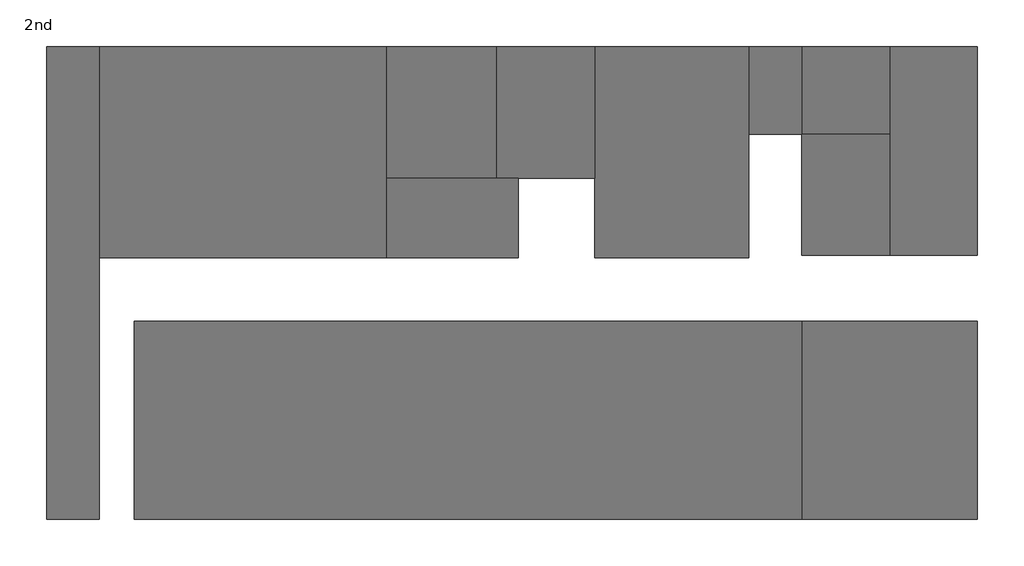
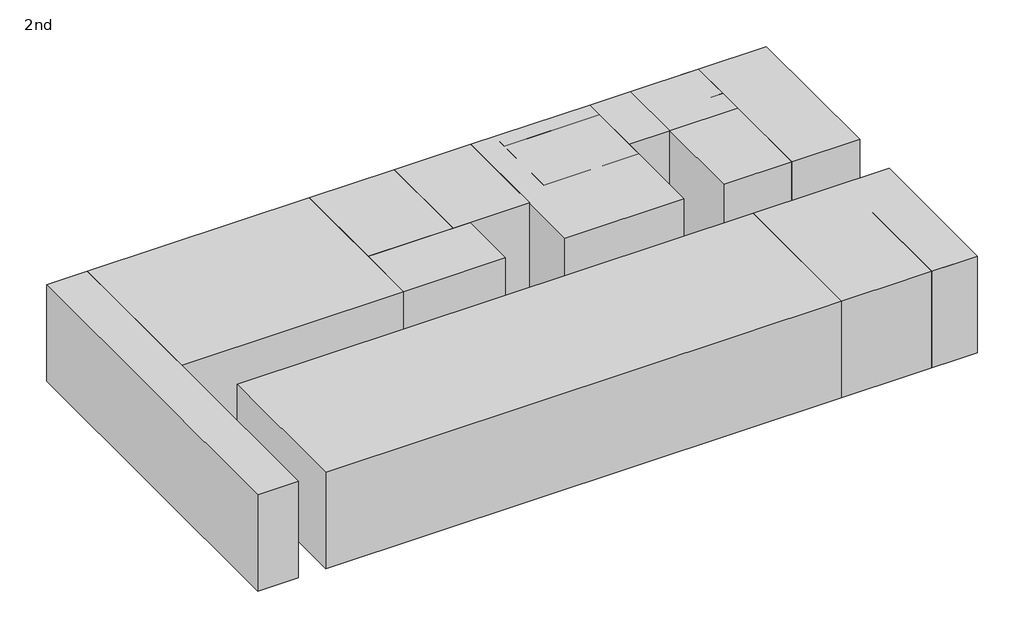
# One storey: 17 proxies.
"""IFC4 building model written with IfcOpenShell, lengths in millimetres."""

import ifcopenshell
import ifcopenshell.guid

model = None  # the IFC model being written
_history = None  # IfcOwnerHistory: only IFC2X3 demands one
_inside = {}  # id of a spatial element -> (the spatial element, [elements in it])
_under = {}  # id of a project, library or spatial element -> (it, [spatial elements below it])
_declared = {}  # id of a project -> (the project, [libraries it declares])
_typed = {}  # id of a type object -> (the type object, [elements of that type])
_made_of = {}  # id of a material, layer set ... -> (it, [elements and type objects made of it])


def new_model(schema):
    """Start an empty IFC model of exactly this schema.

    Asked for "IFC4X3", IfcOpenShell would pick the latest addendum, in which some entities
    have other attributes; the version numbers below select the first issue.
    IFC2X3 requires an IfcOwnerHistory on every rooted entity: one is made here for all.
    """
    global model, _history
    if schema == "IFC4X3":
        model = ifcopenshell.file(schema_version=(4, 3, 0, 0))
    else:
        model = ifcopenshell.file(schema=schema)
    _inside.clear()
    _under.clear()
    _declared.clear()
    _typed.clear()
    _made_of.clear()
    _history = None
    if model.schema == "IFC2X3":
        org = make("IfcOrganization", Name="unknown")
        user = make(
            "IfcPersonAndOrganization",
            ThePerson=make("IfcPerson", FamilyName="unknown"),
            TheOrganization=org,
        )
        app = make(
            "IfcApplication",
            ApplicationDeveloper=org,
            Version="unknown",
            ApplicationFullName="unknown",
            ApplicationIdentifier="unknown",
        )
        _history = make(
            "IfcOwnerHistory",
            OwningUser=user,
            OwningApplication=app,
            ChangeAction="ADDED",
            CreationDate=0,
        )
    return model


def make(cls, **values):
    """One entity of the class cls with the attributes given. An attribute that is None is left unset."""
    return model.create_entity(
        cls, **{name: value for name, value in values.items() if value is not None}
    )


def rooted(cls, **values):
    """An entity with a GlobalId (a new one), such as an element, a storey or a relation."""
    return make(cls, GlobalId=ifcopenshell.guid.new(), OwnerHistory=_history, **values)


def si_unit(unit_type, name, prefix=None):
    """IfcSIUnit, for example si_unit("LENGTHUNIT", "METRE", prefix="MILLI")."""
    return make("IfcSIUnit", UnitType=unit_type, Prefix=prefix, Name=name)


def assignment(units):
    """IfcUnitAssignment: the units of a project."""
    return None if units is None else make("IfcUnitAssignment", Units=units)


def point(xyz):
    """IfcCartesianPoint."""
    return None if xyz is None else make("IfcCartesianPoint", Coordinates=xyz)


def direction(xyz):
    """IfcDirection."""
    return None if xyz is None else make("IfcDirection", DirectionRatios=xyz)


def frame(location, z_axis=None, x_axis=None):
    """IfcAxis2Placement3D, a coordinate frame: its origin and axes. An axis left out is left unset."""
    return make(
        "IfcAxis2Placement3D",
        Location=point(location),
        Axis=direction(z_axis),
        RefDirection=direction(x_axis),
    )


def origin():
    """The frame at (0, 0, 0) with its axes left unset."""
    return frame((0.0, 0.0, 0.0))


def origin_with_axes():
    """The frame at (0, 0, 0) with the z axis (0, 0, 1) and the x axis (1, 0, 0) written out."""
    return frame((0.0, 0.0, 0.0), z_axis=(0.0, 0.0, 1.0), x_axis=(1.0, 0.0, 0.0))


def place(relative_to, where):
    """IfcLocalPlacement: puts the frame where relative to a parent placement (None: the world)."""
    return make(
        "IfcLocalPlacement", PlacementRelTo=relative_to, RelativePlacement=where
    )


def context(
    kind, dimensions, precision=None, world=None, true_north=None, identifier=None
):
    """IfcGeometricRepresentationContext, for example the 3D "Model" context."""
    return make(
        "IfcGeometricRepresentationContext",
        ContextIdentifier=identifier,
        ContextType=kind,
        CoordinateSpaceDimension=dimensions,
        Precision=precision,
        WorldCoordinateSystem=world,
        TrueNorth=true_north,
    )


def project(units=None, contexts=None):
    """IfcProject with its units and contexts."""
    return rooted(
        "IfcProject",
        Name="project",
        RepresentationContexts=contexts,
        UnitsInContext=assignment(units),
    )


def spatial(cls, under=None, at=None, **own):
    """A site, building, storey or space (cls), placed at a placement, below another one or the project."""
    s = rooted(cls, ObjectPlacement=at, **own)
    if under is not None:
        _under.setdefault(under.id(), (under, []))[1].append(s)
    return s


def polyline(points):
    """IfcPolyline through the points."""
    return make("IfcPolyline", Points=[point(p) for p in points])


def outline(outer, holes=None, kind="AREA"):
    """IfcArbitraryClosedProfileDef: a profile drawn as a closed curve; with holes, ...WithVoids."""
    if holes is None:
        return make("IfcArbitraryClosedProfileDef", ProfileType=kind, OuterCurve=outer)
    return make(
        "IfcArbitraryProfileDefWithVoids",
        ProfileType=kind,
        OuterCurve=outer,
        InnerCurves=holes,
    )


def extrude(swept, where, along, depth):
    """IfcExtrudedAreaSolid: the profile swept, set in the frame where, extruded along a direction by depth."""
    return make(
        "IfcExtrudedAreaSolid",
        SweptArea=swept,
        Position=where,
        ExtrudedDirection=direction(along),
        Depth=depth,
    )


def shape(context_of_items, identifier, shape_type, items):
    """IfcShapeRepresentation: the items that make up one representation, for example the "Body"."""
    return make(
        "IfcShapeRepresentation",
        ContextOfItems=context_of_items,
        RepresentationIdentifier=identifier,
        RepresentationType=shape_type,
        Items=items,
    )


def source(mapping_origin, context_of_items, identifier, shape_type, items):
    """IfcRepresentationMap: a shape defined once, which mapped items show again and again."""
    return make(
        "IfcRepresentationMap",
        MappingOrigin=mapping_origin,
        MappedRepresentation=shape(context_of_items, identifier, shape_type, items),
    )


def transform(
    local_origin,
    x_axis=None,
    y_axis=None,
    z_axis=None,
    scale=None,
    scale2=None,
    scale3=None,
    uniform=True,
):
    """IfcCartesianTransformationOperator3D, or its non-uniform kind. x_axis, y_axis, z_axis: its Axis1, 2, 3."""
    if uniform:
        return make(
            "IfcCartesianTransformationOperator3D",
            Axis1=direction(x_axis),
            Axis2=direction(y_axis),
            LocalOrigin=point(local_origin),
            Scale=scale,
            Axis3=direction(z_axis),
        )
    return make(
        "IfcCartesianTransformationOperator3DnonUniform",
        Axis1=direction(x_axis),
        Axis2=direction(y_axis),
        LocalOrigin=point(local_origin),
        Scale=scale,
        Axis3=direction(z_axis),
        Scale2=scale2,
        Scale3=scale3,
    )


def mapped(mapping_source, mapping_target):
    """IfcMappedItem: shows the shape of a source again, moved by a transform."""
    return make(
        "IfcMappedItem", MappingSource=mapping_source, MappingTarget=mapping_target
    )


def made_of(thing, what):
    """Note that an element or type object is made of a material, layer set ...; save() writes the relation."""
    if what is not None:
        _made_of.setdefault(what.id(), (what, []))[1].append(thing)
    return thing


def element(
    cls,
    number,
    at=None,
    inside=None,
    cuts=None,
    type_object=None,
    material=None,
    context=None,
    identifier="Body",
    shape_type=None,
    held_by="IfcProductDefinitionShape",
    body=None,
    shapes=None,
    **own,
):
    """One element of the class cls, such as IfcWall. Its Tag is "e" and its number.

    at: its placement. inside: the storey or other place that contains it. cuts: it is an
    opening in that element (IfcRelVoidsElement). A single representation is given by context,
    identifier, shape_type and body (its items); several are given by shapes. held_by: the class
    of the entity that holds the representations. save() writes the other relations.
    """
    e = rooted(cls, Tag="e%d" % number, ObjectPlacement=at, **own)
    if body is not None:
        shapes = [shape(context, identifier, shape_type, body)]
    if shapes is not None:
        e.Representation = make(held_by, Representations=shapes)
    if inside is not None:
        _inside.setdefault(inside.id(), (inside, []))[1].append(e)
    if cuts is not None:
        rooted(
            "IfcRelVoidsElement", RelatingBuildingElement=cuts, RelatedOpeningElement=e
        )
    if type_object is not None:
        _typed.setdefault(type_object.id(), (type_object, []))[1].append(e)
    return made_of(e, material)


def aggregate(whole, parts):
    """IfcRelAggregates: a whole, such as a stair, and the parts it consists of."""
    return rooted("IfcRelAggregates", RelatingObject=whole, RelatedObjects=parts)


def save(model, path):
    """Write the relations noted so far, then the file.

    IfcRelAggregates (storeys below a building ...), IfcRelContainedInSpatialStructure (elements
    in a storey), IfcRelDefinesByType, IfcRelAssociatesMaterial and IfcRelDeclares: one each for
    every whole, place, type object, material and project.
    """
    for whole, parts in _under.values():
        aggregate(whole, parts)
    for where, things in _inside.values():
        rooted(
            "IfcRelContainedInSpatialStructure",
            RelatedElements=things,
            RelatingStructure=where,
        )
    for kind, things in _typed.values():
        rooted("IfcRelDefinesByType", RelatedObjects=things, RelatingType=kind)
    for what, things in _made_of.values():
        rooted("IfcRelAssociatesMaterial", RelatedObjects=things, RelatingMaterial=what)
    for by, libraries in _declared.values():
        rooted("IfcRelDeclares", RelatingContext=by, RelatedDefinitions=libraries)
    model.write(path)


def space_planning_box_space_planning_box_5634f436(model_context):
    return source(origin(), model_context, "Body", "SweptSolid", [
        extrude(outline(polyline([(1350.0, 3000.0), (1350.0, -3000.0), (-1350.0, -3000.0), (-1350.0, 3000.0), (1350.0, 3000.0)])), origin_with_axes(), (0.0, 0.0, 1.0), 6000.0),
    ])


def space_planning_box_space_planning_box_71e2440f(model_context):
    return source(origin(), model_context, "Body", "SweptSolid", [
        extrude(outline(polyline([(500.0, 1250.0), (500.0, -1250.0), (-500.0, -1250.0), (-500.0, 1250.0), (500.0, 1250.0)])), origin_with_axes(), (0.0, 0.0, 1.0), 6000.0),
    ])


def space_planning_box_space_planning_box_ce7d2093(model_context):
    return source(origin(), model_context, "Body", "SweptSolid", [
        extrude(outline(polyline([(4500.0, 15175.0), (4500.0, -15175.0), (-4500.0, -15175.0), (-4500.0, 15175.0), (4500.0, 15175.0)])), origin_with_axes(), (0.0, 0.0, 1.0), 6000.0),
    ])


def space_planning_box_space_planning_box_c2e9f8fb(model_context):
    return source(origin(), model_context, "Body", "SweptSolid", [
        extrude(outline(polyline([(4800.0, 6525.0), (4800.0, -6525.0), (-4800.0, -6525.0), (-4800.0, 6525.0), (4800.0, 6525.0)])), origin_with_axes(), (0.0, 0.0, 1.0), 6000.0),
    ])


def space_planning_box_space_planning_box_44ef6168(model_context):
    return source(origin(), model_context, "Body", "SweptSolid", [
        extrude(outline(polyline([(2500.0, 3000.0), (2500.0, -3000.0), (-2500.0, -3000.0), (-2500.0, 3000.0), (2500.0, 3000.0)])), origin_with_axes(), (0.0, 0.0, 1.0), 6000.0),
    ])


def space_planning_box_space_planning_box_4d084078(model_context):
    return source(origin(), model_context, "Body", "SweptSolid", [
        extrude(outline(polyline([(4000.0, 4500.0), (4000.0, -4500.0), (-4000.0, -4500.0), (-4000.0, 4500.0), (4000.0, 4500.0)])), origin_with_axes(), (0.0, 0.0, 1.0), 6000.0),
    ])


def space_planning_box_space_planning_box_072414e0(model_context):
    return source(origin(), model_context, "Body", "SweptSolid", [
        extrude(outline(polyline([(3500.0, 4800.0), (3500.0, -4800.0), (-3500.0, -4800.0), (-3500.0, 4800.0), (3500.0, 4800.0)])), origin_with_axes(), (0.0, 0.0, 1.0), 6000.0),
    ])


def space_planning_box_space_planning_box_34e84c64(model_context):
    return source(origin(), model_context, "Body", "SweptSolid", [
        extrude(outline(polyline([(2750.0, 2000.0), (2750.0, -2000.0), (-2750.0, -2000.0), (-2750.0, 2000.0), (2750.0, 2000.0)])), origin_with_axes(), (0.0, 0.0, 1.0), 6000.0),
    ])


def space_planning_box_space_planning_box_7bff30ad(model_context):
    return source(origin(), model_context, "Body", "SweptSolid", [
        extrude(outline(polyline([(2000.0, 2000.0), (2000.0, -2000.0), (-2000.0, -2000.0), (-2000.0, 2000.0), (2000.0, 2000.0)])), origin_with_axes(), (0.0, 0.0, 1.0), 6000.0),
    ])


def space_planning_box_space_planning_box_03407eb8(model_context):
    return source(origin(), model_context, "Body", "SweptSolid", [
        extrude(outline(polyline([(1200.0, 10750.0), (1200.0, -10750.0), (-1200.0, -10750.0), (-1200.0, 10750.0), (1200.0, 10750.0)])), origin_with_axes(), (0.0, 0.0, 1.0), 6000.0),
    ])


def space_planning_box_space_planning_box_3a820573(model_context):
    return source(origin(), model_context, "Body", "SweptSolid", [
        extrude(outline(polyline([(2000.0, 4750.0), (2000.0, -4750.0), (-2000.0, -4750.0), (-2000.0, 4750.0), (2000.0, 4750.0)])), origin_with_axes(), (0.0, 0.0, 1.0), 6000.0),
    ])


def space_planning_box_space_planning_box_8af91fed(model_context):
    return source(origin(), model_context, "Body", "SweptSolid", [
        extrude(outline(polyline([(2250.0, 3000.0), (2250.0, -3000.0), (-2250.0, -3000.0), (-2250.0, 3000.0), (2250.0, 3000.0)])), origin_with_axes(), (0.0, 0.0, 1.0), 6000.0),
    ])


def space_planning_box_space_planning_box_837d2e24(model_context):
    return source(origin(), model_context, "Body", "SweptSolid", [
        extrude(outline(polyline([(1800.0, 3000.0), (1800.0, -3000.0), (-1800.0, -3000.0), (-1800.0, 3000.0), (1800.0, 3000.0)])), origin_with_axes(), (0.0, 0.0, 1.0), 6000.0),
    ])


def space_planning_box_space_planning_box_47b98be1(model_context):
    return source(origin(), model_context, "Body", "SweptSolid", [
        extrude(outline(polyline([(1200.0, 2000.0), (1200.0, -2000.0), (-1200.0, -2000.0), (-1200.0, 2000.0), (1200.0, 2000.0)])), origin_with_axes(), (0.0, 0.0, 1.0), 6000.0),
    ])


def space_planning_box_space_planning_box_a556ef48(model_context):
    return source(origin(), model_context, "Body", "SweptSolid", [
        extrude(outline(polyline([(500.0, 2800.0), (500.0, -2800.0), (-500.0, -2800.0), (-500.0, 2800.0), (500.0, 2800.0)])), origin_with_axes(), (0.0, 0.0, 1.0), 6000.0),
    ])


def space_planning_box_space_planning_box_c1734578(model_context):
    return source(origin(), model_context, "Body", "SweptSolid", [
        extrude(outline(polyline([(2800.0, 2500.0), (2800.0, -2500.0), (-2800.0, -2500.0), (-2800.0, 2500.0), (2800.0, 2500.0)])), origin_with_axes(), (0.0, 0.0, 1.0), 6000.0),
    ])


model = new_model("IFC4")

# Units and contexts
model_context = context("Model", 3, world=origin())
ifc_project = project(units=[si_unit("LENGTHUNIT", "METRE", prefix="MILLI")], contexts=[model_context])

# Site, building, storey
site = spatial("IfcSite", under=ifc_project)
building = spatial("IfcBuilding", under=site)
storey = spatial("IfcBuildingStorey", under=building, Name="2nd", Elevation=14000.0)

# Proxies
placement = place(None, origin())
space_planning_box_space_planning_box_shape = space_planning_box_space_planning_box_5634f436(model_context)
element("IfcBuildingElementProxy", 1, Name="Space Planning Box : Space Planning Box", ObjectType="Space Planning Box : Space Planning Box", at=placement, inside=storey, context=model_context, shape_type="MappedRepresentation", body=[
    mapped(space_planning_box_space_planning_box_shape, transform((48750.0, 154250.0, 14000.0), x_axis=(1.0, 0.0, 0.0), y_axis=(0.0, 1.0, 0.0), z_axis=(0.0, 0.0, 1.0))),
])
space_planning_box_space_planning_box_2_shape = space_planning_box_space_planning_box_71e2440f(model_context)
element("IfcBuildingElementProxy", 2, Name="Space Planning Box : Space Planning Box", ObjectType="Space Planning Box : Space Planning Box", at=placement, inside=storey, context=model_context, shape_type="MappedRepresentation", body=[
    mapped(space_planning_box_space_planning_box_2_shape, transform((45600.0, 171500.0, 14000.0), x_axis=(1.0, 0.0, 0.0), y_axis=(0.0, 1.0, 0.0), z_axis=(0.0, 0.0, 1.0))),
])
space_planning_box_space_planning_box_3_shape = space_planning_box_space_planning_box_ce7d2093(model_context)
element("IfcBuildingElementProxy", 3, Name="Space Planning Box : Space Planning Box", ObjectType="Space Planning Box : Space Planning Box", at=placement, inside=storey, context=model_context, shape_type="MappedRepresentation", body=[
    mapped(space_planning_box_space_planning_box_3_shape, transform((26925.0, 155750.0, 14000.0), x_axis=(0.0, -1.0, 0.0), y_axis=(1.0, 0.0, 0.0), z_axis=(0.0, 0.0, 1.0))),
])
space_planning_box_space_planning_box_4_shape = space_planning_box_space_planning_box_c2e9f8fb(model_context)
element("IfcBuildingElementProxy", 4, Name="Space Planning Box : Space Planning Box", ObjectType="Space Planning Box : Space Planning Box", at=placement, inside=storey, context=model_context, shape_type="MappedRepresentation", body=[
    mapped(space_planning_box_space_planning_box_4_shape, transform((16675.0, 167950.0, 14000.0), x_axis=(0.0, -1.0, 0.0), y_axis=(1.0, 0.0, 0.0), z_axis=(0.0, 0.0, 1.0))),
])
space_planning_box_space_planning_box_5_shape = space_planning_box_space_planning_box_44ef6168(model_context)
element("IfcBuildingElementProxy", 5, Name="Space Planning Box : Space Planning Box", ObjectType="Space Planning Box : Space Planning Box", at=placement, inside=storey, context=model_context, shape_type="MappedRepresentation", body=[
    mapped(space_planning_box_space_planning_box_5_shape, transform((25700.0, 169750.0, 14000.0), x_axis=(1.0, 0.0, 0.0), y_axis=(0.0, 1.0, 0.0), z_axis=(0.0, 0.0, 1.0))),
])
space_planning_box_space_planning_box_6_shape = space_planning_box_space_planning_box_4d084078(model_context)
element("IfcBuildingElementProxy", 6, Name="Space Planning Box : Space Planning Box", ObjectType="Space Planning Box : Space Planning Box", at=placement, inside=storey, context=model_context, shape_type="MappedRepresentation", body=[
    mapped(space_planning_box_space_planning_box_6_shape, transform((46100.0, 155750.0, 14000.0), x_axis=(1.0, 0.0, 0.0), y_axis=(0.0, 1.0, 0.0), z_axis=(0.0, 0.0, 1.0))),
])
space_planning_box_space_planning_box_7_shape = space_planning_box_space_planning_box_072414e0(model_context)
element("IfcBuildingElementProxy", 7, Name="Space Planning Box : Space Planning Box", ObjectType="Space Planning Box : Space Planning Box", at=placement, inside=storey, context=model_context, shape_type="MappedRepresentation", body=[
    mapped(space_planning_box_space_planning_box_7_shape, transform((36200.0, 167950.0, 14000.0), x_axis=(1.0, 0.0, 0.0), y_axis=(0.0, 1.0, 0.0), z_axis=(0.0, 0.0, 1.0))),
])
space_planning_box_space_planning_box_8_shape = space_planning_box_space_planning_box_34e84c64(model_context)
element("IfcBuildingElementProxy", 8, Name="Space Planning Box : Space Planning Box", ObjectType="Space Planning Box : Space Planning Box", at=placement, inside=storey, context=model_context, shape_type="MappedRepresentation", body=[
    mapped(space_planning_box_space_planning_box_8_shape, transform((44100.0, 166000.0, 14000.0), x_axis=(0.0, -1.0, 0.0), y_axis=(1.0, 0.0, 0.0), z_axis=(0.0, 0.0, 1.0))),
])
space_planning_box_space_planning_box_9_shape = space_planning_box_space_planning_box_7bff30ad(model_context)
element("IfcBuildingElementProxy", 9, Name="Space Planning Box : Space Planning Box", ObjectType="Space Planning Box : Space Planning Box", at=placement, inside=storey, context=model_context, shape_type="MappedRepresentation", body=[
    mapped(space_planning_box_space_planning_box_9_shape, transform((44100.0, 170750.0, 14000.0), x_axis=(1.0, 0.0, 0.0), y_axis=(0.0, 1.0, 0.0), z_axis=(0.0, 0.0, 1.0))),
])
space_planning_box_space_planning_box_10_shape = space_planning_box_space_planning_box_03407eb8(model_context)
element("IfcBuildingElementProxy", 10, Name="Space Planning Box : Space Planning Box", ObjectType="Space Planning Box : Space Planning Box", at=placement, inside=storey, context=model_context, shape_type="MappedRepresentation", body=[
    mapped(space_planning_box_space_planning_box_10_shape, transform((8950.0, 162000.0, 14000.0), x_axis=(1.0, 0.0, 0.0), y_axis=(0.0, 1.0, 0.0), z_axis=(0.0, 0.0, 1.0))),
])
space_planning_box_space_planning_box_11_shape = space_planning_box_space_planning_box_3a820573(model_context)
element("IfcBuildingElementProxy", 11, Name="Space Planning Box : Space Planning Box", ObjectType="Space Planning Box : Space Planning Box", at=placement, inside=storey, context=model_context, shape_type="MappedRepresentation", body=[
    mapped(space_planning_box_space_planning_box_11_shape, transform((48100.0, 168000.0, 14000.0), x_axis=(1.0, 0.0, 0.0), y_axis=(0.0, 1.0, 0.0), z_axis=(0.0, 0.0, 1.0))),
])
space_planning_box_space_planning_box_12_shape = space_planning_box_space_planning_box_8af91fed(model_context)
element("IfcBuildingElementProxy", 12, Name="Space Planning Box : Space Planning Box", ObjectType="Space Planning Box : Space Planning Box", at=placement, inside=storey, context=model_context, shape_type="MappedRepresentation", body=[
    mapped(space_planning_box_space_planning_box_12_shape, transform((30450.0, 169750.0, 14000.0), x_axis=(1.0, 0.0, 0.0), y_axis=(0.0, 1.0, 0.0), z_axis=(0.0, 0.0, 1.0))),
])
space_planning_box_space_planning_box_13_shape = space_planning_box_space_planning_box_837d2e24(model_context)
element("IfcBuildingElementProxy", 13, Name="Space Planning Box : Space Planning Box", ObjectType="Space Planning Box : Space Planning Box", at=placement, inside=storey, context=model_context, shape_type="MappedRepresentation", body=[
    mapped(space_planning_box_space_planning_box_13_shape, transform((26200.0, 164950.0, 14000.0), x_axis=(0.0, -1.0, 0.0), y_axis=(1.0, 0.0, 0.0), z_axis=(0.0, 0.0, 1.0))),
])
space_planning_box_space_planning_box_14_shape = space_planning_box_space_planning_box_47b98be1(model_context)
element("IfcBuildingElementProxy", 14, Name="Space Planning Box : Space Planning Box", ObjectType="Space Planning Box : Space Planning Box", at=placement, inside=storey, context=model_context, shape_type="MappedRepresentation", body=[
    mapped(space_planning_box_space_planning_box_14_shape, transform((40900.0, 170750.0, 14000.0), x_axis=(1.0, 0.0, 0.0), y_axis=(0.0, 1.0, 0.0), z_axis=(0.0, 0.0, 1.0))),
])
element("IfcBuildingElementProxy", 15, Name="Space Planning Box : Space Planning Box", ObjectType="Space Planning Box : Space Planning Box", at=placement, inside=storey, context=model_context, shape_type="MappedRepresentation", body=[
    mapped(space_planning_box_space_planning_box_14_shape, transform((40900.0, 170750.0, 14000.0), x_axis=(1.0, 0.0, 0.0), y_axis=(0.0, 1.0, 0.0), z_axis=(0.0, 0.0, 1.0))),
])
space_planning_box_space_planning_box_15_shape = space_planning_box_space_planning_box_a556ef48(model_context)
element("IfcBuildingElementProxy", 16, Name="Space Planning Box : Space Planning Box", ObjectType="Space Planning Box : Space Planning Box", at=placement, inside=storey, context=model_context, shape_type="MappedRepresentation", body=[
    mapped(space_planning_box_space_planning_box_15_shape, transform((36900.0, 172250.0, 14000.0), x_axis=(0.0, 1.0, 0.0), y_axis=(-1.0, 0.0, 0.0), z_axis=(0.0, 0.0, 1.0))),
])
space_planning_box_space_planning_box_16_shape = space_planning_box_space_planning_box_c1734578(model_context)
element("IfcBuildingElementProxy", 17, Name="Space Planning Box : Space Planning Box", ObjectType="Space Planning Box : Space Planning Box", at=placement, inside=storey, context=model_context, shape_type="MappedRepresentation", body=[
    mapped(space_planning_box_space_planning_box_16_shape, transform((36900.0, 170250.0, 14000.0), x_axis=(1.0, 0.0, 0.0), y_axis=(0.0, 1.0, 0.0), z_axis=(0.0, 0.0, 1.0))),
])

save(model, "model.ifc")

# Revit data of these elements
# Project information
#   Project Issue Date = "Issue Date"
#   Project Status = "Project Status"
#   Client Name = "Owner"
#   Project Address = "Enter address here"
#   Project Name = "Project Name"
#   Project Number = "Project Number"
# Type "Space Planning Box : Space Planning Box"
#   Type Comments = "..."
#   Room Name [instance default] = "?"
#   Assembly Code = "..."
#   Width [instance default] = 1524 mm
#   Program Area [instance default] = 0 m²
#   Length [instance default] = 1524 mm
#   Height [instance default] = 1524 mm
#   Area [instance default] = 2.32258 m²
#   Fill Color [instance default] = Cyan
#   Default Elevation = 0
# Element 1 (IfcBuildingElementProxy, "Space Planning Box : Space Planning Box")
#   Room Name = "Duct Shaft"
#   Width = 2700 mm
#   Program Area = 16.2 m²
#   Length = 6000 mm
#   Height = 6000 mm
#   Area = 16.2 m²
#   Fill Color = Pink
#   Phase Created = New Construction
#   Materials on its faces: "Pink"
# Element 2 (IfcBuildingElementProxy, "Space Planning Box : Space Planning Box")
#   Room Name = "Pipe Shaft"
#   Width = 1000 mm
#   Program Area = 2.5 m²
#   Length = 2500 mm
#   Height = 6000 mm
#   Area = 2.5 m²
#   Fill Color = Pink
#   Phase Created = New Construction
#   Materials on its faces: "Pink"
# Element 3 (IfcBuildingElementProxy, "Space Planning Box : Space Planning Box")
#   Room Name = "Central Control Room"
#   Width = 9000 mm
#   Program Area = 288 m²
#   Length = 30350 mm
#   Height = 6000 mm
#   Area = 273.15 m²
#   Fill Color = Lime
#   Phase Created = New Construction
#   Materials on its faces: "Lime"
# Element 4 (IfcBuildingElementProxy, "Space Planning Box : Space Planning Box")
#   Room Name = "Engineer Room"
#   Width = 9600 mm
#   Program Area = 120 m²
#   Length = 13050 mm
#   Height = 6000 mm
#   Area = 125.28 m²
#   Fill Color = Lime
#   Phase Created = New Construction
#   Materials on its faces: "Lime"
# Element 5 (IfcBuildingElementProxy, "Space Planning Box : Space Planning Box")
#   Room Name = "Document Room"
#   Width = 5000 mm
#   Program Area = 48 m²
#   Length = 6000 mm
#   Height = 6000 mm
#   Area = 30 m²
#   Fill Color = Lavender
#   Phase Created = New Construction
#   Materials on its faces: "Lavender"
# Element 6 (IfcBuildingElementProxy, "Space Planning Box : Space Planning Box")
#   Room Name = "Fire Gas Room"
#   Width = 8000 mm
#   Program Area = 0 m²
#   Length = 9000 mm
#   Height = 6000 mm
#   Area = 72 m²
#   Fill Color = Cyan
#   Phase Created = New Construction
#   Materials on its faces: "Cyan"
# Element 7 (IfcBuildingElementProxy, "Space Planning Box : Space Planning Box")
#   Room Name = "Kitch & Lunch Room"
#   Width = 7000 mm
#   Program Area = 31.5 m²
#   Length = 9600 mm
#   Height = 6000 mm
#   Area = 67.2 m²
#   Fill Color = Lavender
#   Phase Created = New Construction
#   Materials on its faces: "Lavender"
# Element 8 (IfcBuildingElementProxy, "Space Planning Box : Space Planning Box")
#   Room Name = "Toilet (M)"
#   Width = 5500 mm
#   Program Area = 72 m²
#   Length = 4000 mm
#   Height = 6000 mm
#   Area = 22 m²
#   Fill Color = Lavender
#   Phase Created = New Construction
#   Materials on its faces: "Lavender"
# Element 9 (IfcBuildingElementProxy, "Space Planning Box : Space Planning Box")
#   Room Name = "Toilet (F)"
#   Width = 4000 mm
#   Program Area = 72 m²
#   Length = 4000 mm
#   Height = 6000 mm
#   Area = 16 m²
#   Fill Color = Lavender
#   Phase Created = New Construction
#   Materials on its faces: "Lavender"
# Element 10 (IfcBuildingElementProxy, "Space Planning Box : Space Planning Box")
#   Room Name = "Corridor"
#   Width = 2400 mm
#   Program Area = 0 m²
#   Length = 21500 mm
#   Height = 6000 mm
#   Area = 51.6 m²
#   Fill Color = Lavender
#   Phase Created = New Construction
#   Materials on its faces: "Lavender"
# Element 11 (IfcBuildingElementProxy, "Space Planning Box : Space Planning Box")
#   Room Name = "Stairway"
#   Width = 4000 mm
#   Program Area = 38 m²
#   Length = 9500 mm
#   Height = 6000 mm
#   Area = 38 m²
#   Fill Color = Lavender
#   Phase Created = New Construction
#   Materials on its faces: "Lavender"
# Element 12 (IfcBuildingElementProxy, "Space Planning Box : Space Planning Box")
#   Room Name = "Shift Office Room"
#   Width = 4500 mm
#   Program Area = 43.2 m²
#   Length = 6000 mm
#   Height = 6000 mm
#   Area = 27 m²
#   Fill Color = Lavender
#   Phase Created = New Construction
#   Materials on its faces: "Lavender"
# Element 13 (IfcBuildingElementProxy, "Space Planning Box : Space Planning Box")
#   Room Name = "LOTO Office Room"
#   Width = 3600 mm
#   Program Area = 31.5 m²
#   Length = 6000 mm
#   Height = 6000 mm
#   Area = 21.6 m²
#   Fill Color = Lavender
#   Phase Created = New Construction
#   Materials on its faces: "Lavender"
# Element 14 (IfcBuildingElementProxy, "Space Planning Box : Space Planning Box")
#   Room Name = "Shower Room (F)"
#   Width = 2400 mm
#   Program Area = 31.5 m²
#   Length = 4000 mm
#   Height = 6000 mm
#   Area = 9.6 m²
#   Fill Color = Lavender
#   Phase Created = New Construction
#   Materials on its faces: "Lavender"
# Element 15 (IfcBuildingElementProxy, "Space Planning Box : Space Planning Box")
#   Room Name = "Locker Room (F)"
#   Width = 2400 mm
#   Program Area = 31.5 m²
#   Length = 4000 mm
#   Height = 6000 mm
#   Area = 9.6 m²
#   Fill Color = Lavender
#   Phase Created = New Construction
#   Materials on its faces: "Lavender"
# Element 16 (IfcBuildingElementProxy, "Space Planning Box : Space Planning Box")
#   Room Name = "Shower Room (M)"
#   Width = 1000 mm
#   Program Area = 31.5 m²
#   Length = 5600 mm
#   Height = 6000 mm
#   Area = 5.6 m²
#   Fill Color = Lavender
#   Phase Created = New Construction
#   Materials on its faces: "Lavender"
# Element 17 (IfcBuildingElementProxy, "Space Planning Box : Space Planning Box")
#   Room Name = "Locker Room (M)"
#   Width = 5600 mm
#   Program Area = 31.5 m²
#   Length = 5000 mm
#   Height = 6000 mm
#   Area = 28 m²
#   Fill Color = Lavender
#   Phase Created = New Construction
#   Materials on its faces: "Lavender"
# Materials
#   "Cyan": class "Generic", colour RGB 0 255 255, transparency 0.2, Cost = 0
#   "Pink": class "Generic", colour RGB 255 105 180, transparency 0.2, Cost = 0
#   "Lime": class "Generic", colour RGB 0 255 0, transparency 0.2, Cost = 0
#   "Lavender": class "Generic", colour RGB 186 85 211, transparency 0.2, Cost = 0
